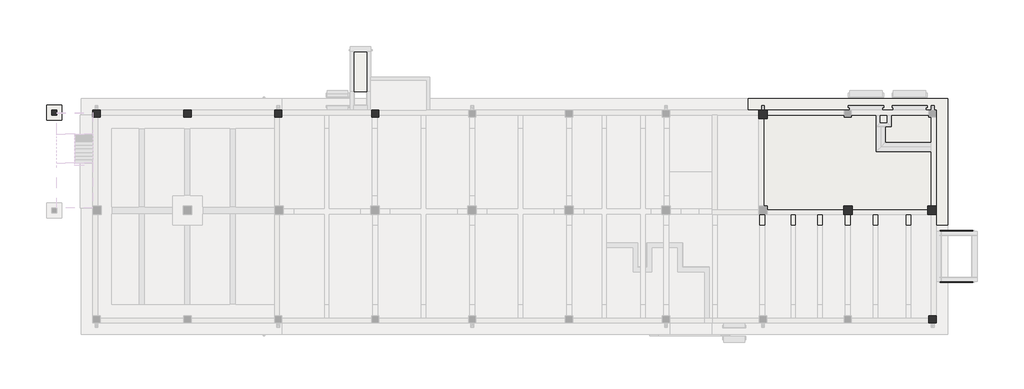
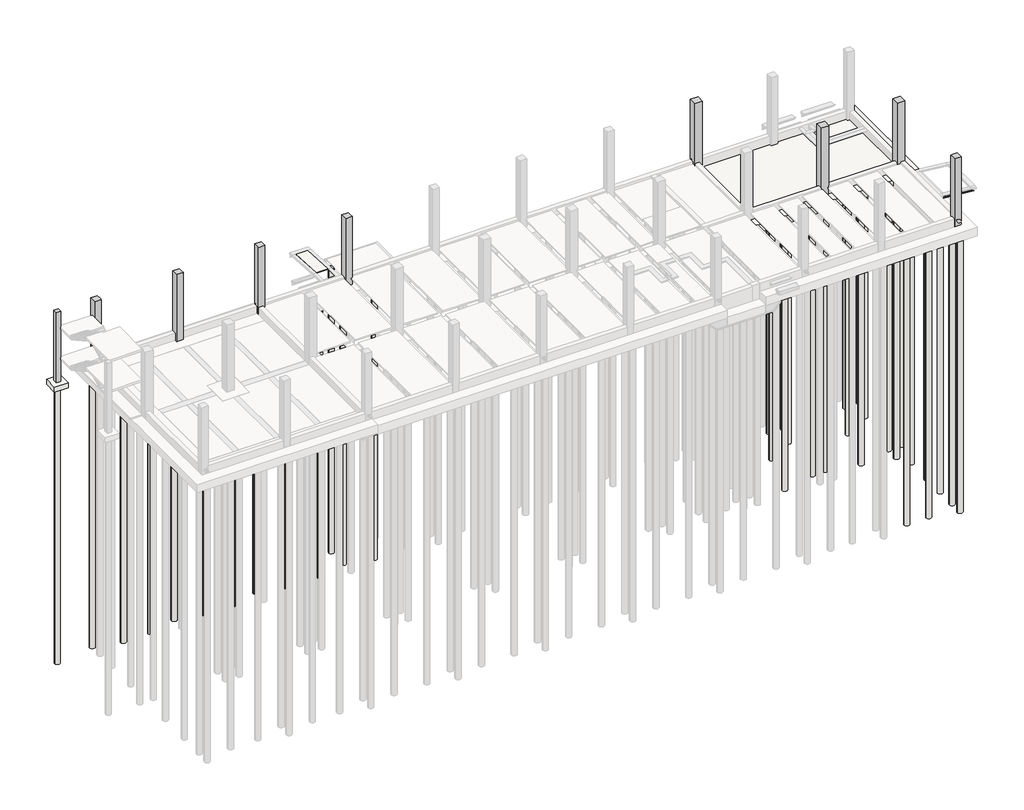
# One storey, part 6 of 7: 46 slabs, 9 columns.
"""IFC4 building model written with IfcOpenShell, lengths in millimetres."""

from ifc_helpers import new_model, si_unit, point, frame, frame_2d, origin, place, context, project, spatial, polyline, circle_curve, trimmed, segment, composite_curve, outline, extrude, faceted_brep, element, save

model = new_model("IFC4")

# Units and contexts
model_context = context("Model", 3, world=origin())
ifc_project = project(units=[si_unit("LENGTHUNIT", "METRE", prefix="MILLI")], contexts=[model_context])

# Site, building, storey
site = spatial("IfcSite", under=ifc_project)
building = spatial("IfcBuilding", under=site)
storey = spatial("IfcBuildingStorey", under=building, Name="H.P.P", Elevation=4500.0)

# Columns
placement = place(None, origin())
element("IfcColumn", 1, ObjectType="RC_Column_Rectangular : H_SC_AR S15_RC Col-AG_700x700_C1", at=placement, inside=storey, context=model_context, shape_type="Brep", body=[
    faceted_brep([(62350.0, -7650.0, 4000.0), (62350.0, -7950.0, 4000.0), (62350.0, -8350.0, 4000.0), (61650.0, -8350.0, 4000.0), (61650.0, -7950.0, 4000.0), (61650.0, -7650.0, 4000.0), (62350.0, -7650.0, 10600.0), (62350.0, -8350.0, 10600.0), (62350.0, -8350.0, 10450.0), (62350.0, -8350.0, 9800.0), (62350.0, -8350.0, 4800.0), (62350.0, -8350.0, 4650.0), (62250.0, -8350.0, 10600.0), (61750.0, -8350.0, 10600.0), (61650.0, -8350.0, 10600.0), (61650.0, -8350.0, 10450.0), (61650.0, -8350.0, 9800.0), (61650.0, -8350.0, 4800.0), (61650.0, -8350.0, 4650.0), (61650.0, -7650.0, 10600.0)], [[[0, 1, 2, 3, 4, 5]], [[2, 1, 0, 6, 7, 8, 9, 10, 11]], [[3, 2, 11, 10, 9, 8, 7, 12, 13, 14, 15, 16, 17, 18]], [[5, 4, 3, 18, 17, 16, 15, 14, 19]], [[0, 5, 19, 6]], [[7, 6, 19, 14, 13, 12]]]),
])
element("IfcColumn", 2, ObjectType="RC_Column_Rectangular : H_SC_AR S15_RC Col-AG_700x700_C1", at=placement, inside=storey, context=model_context, shape_type="Brep", body=[
    faceted_brep([(69300.0, -7650.0, 4000.0), (69300.0, -8350.0, 4000.0), (68900.0, -8350.0, 4000.0), (68600.0, -8350.0, 4000.0), (68600.0, -7950.0, 4000.0), (68600.0, -7650.0, 4000.0), (68900.0, -7650.0, 4000.0), (69300.0, -7650.0, 4800.0), (69300.0, -7650.0, 9900.0), (69300.0, -7650.0, 10600.0), (69300.0, -8350.0, 10600.0), (69300.0, -8350.0, 9900.0), (69300.0, -8350.0, 4800.0), (68900.0, -8350.0, 10600.0), (68600.0, -8350.0, 10600.0), (68600.0, -8350.0, 10450.0), (68600.0, -8350.0, 9800.0), (68600.0, -8350.0, 4800.0), (68600.0, -8350.0, 4650.0), (68600.0, -7650.0, 10600.0), (68900.0, -7650.0, 10600.0)], [[[0, 1, 2, 3, 4, 5, 6]], [[1, 0, 7, 8, 9, 10, 11, 12]], [[3, 2, 1, 12, 11, 10, 13, 14, 15, 16, 17, 18]], [[5, 4, 3, 18, 17, 16, 15, 14, 19]], [[0, 6, 5, 19, 20, 9, 8, 7]], [[10, 9, 20, 19, 14, 13]]]),
])
element("IfcColumn", 3, ObjectType="RC_Column_Rectangular : H_SC_AR S15_RC Col-AG_700x700_C1", at=placement, inside=storey, context=model_context, shape_type="Brep", body=[
    faceted_brep([(55350.0, 300.0, 4000.0), (55350.0, -100.0, 4000.0), (55350.0, -400.0, 4000.0), (55050.0, -400.0, 4000.0), (54650.0, -400.0, 4000.0), (54650.0, -100.0, 4000.0), (54650.0, 300.0, 4000.0), (55350.0, 300.0, 10600.0), (55350.0, -400.0, 10600.0), (55350.0, 300.0, 4800.0), (55350.0, 300.0, 8300.0), (55350.0, 300.0, 9100.0), (54650.0, -400.0, 10600.0), (54650.0, -400.0, 9800.0), (54650.0, -400.0, 4800.0), (54650.0, 300.0, 10600.0), (54650.0, 300.0, 9800.0), (54650.0, 300.0, 4800.0)], [[[0, 1, 2, 3, 4, 5, 6]], [[7, 8, 2, 1, 0, 9, 10, 11]], [[8, 12, 13, 14, 4, 3, 2]], [[12, 15, 16, 17, 6, 5, 4, 14, 13]], [[15, 7, 11, 10, 9, 0, 6, 17, 16]], [[7, 15, 12, 8]]]),
])
element("IfcColumn", 4, ObjectType="RC_Column_Rectangular : H_SC_AR S15_RC Col-AG_600x600_C2", at=placement, inside=storey, context=model_context, shape_type="Brep", body=[
    faceted_brep([(300.0, 300.0, 4100.0), (300.0, -100.0, 4100.0), (300.0, -300.0, 4100.0), (100.0, -300.0, 4100.0), (-300.0, -300.0, 4100.0), (-300.0, -100.0, 4100.0), (-300.0, 300.0, 4100.0), (300.0, 300.0, 4800.0), (300.0, 300.0, 9800.0), (300.0, 300.0, 10600.0), (300.0, -100.0, 10600.0), (300.0, -300.0, 10600.0), (300.0, -300.0, 10450.0), (100.0, -300.0, 10600.0), (-300.0, -300.0, 10600.0), (-300.0, -300.0, 9900.0), (-300.0, -300.0, 4800.0), (-300.0, 300.0, 10600.0), (-300.0, 300.0, 10550.0), (-300.0, 300.0, 9950.0), (-300.0, 300.0, 4630.0)], [[[0, 1, 2, 3, 4, 5, 6]], [[2, 1, 0, 7, 8, 9, 10, 11, 12]], [[4, 3, 2, 12, 11, 13, 14, 15, 16]], [[6, 5, 4, 16, 15, 14, 17, 18, 19, 20]], [[0, 6, 20, 19, 18, 17, 9, 8, 7]], [[17, 14, 13, 11, 10, 9]]]),
])
element("IfcColumn", 5, ObjectType="RC_Column_Rectangular : H_SC_AR S15_RC Col-AG_600x600_C2", at=placement, inside=storey, context=model_context, shape_type="Brep", body=[
    faceted_brep([(7800.0, 300.0, 4100.0), (7800.0, -100.0, 4100.0), (7800.0, -300.0, 4100.0), (7200.0, -300.0, 4100.0), (7200.0, -100.0, 4100.0), (7200.0, 300.0, 4100.0), (7800.0, 300.0, 4800.0), (7800.0, 300.0, 9800.0), (7800.0, 300.0, 10600.0), (7800.0, -100.0, 10600.0), (7800.0, -300.0, 10600.0), (7800.0, -300.0, 10450.0), (7750.0, -300.0, 10600.0), (7250.0, -300.0, 10600.0), (7200.0, -300.0, 10600.0), (7200.0, -300.0, 10450.0), (7200.0, -100.0, 10600.0), (7200.0, 300.0, 10600.0), (7200.0, 300.0, 9800.0), (7200.0, 300.0, 4800.0)], [[[0, 1, 2, 3, 4, 5]], [[2, 1, 0, 6, 7, 8, 9, 10, 11]], [[3, 2, 11, 10, 12, 13, 14, 15]], [[5, 4, 3, 15, 14, 16, 17, 18, 19]], [[0, 5, 19, 18, 17, 8, 7, 6]], [[8, 17, 16, 14, 13, 12, 10, 9]]]),
])
element("IfcColumn", 6, ObjectType="RC_Column_Rectangular : H_SC_AR S15_RC Col-AG_600x600_C2", at=placement, inside=storey, context=model_context, shape_type="Brep", body=[
    faceted_brep([(15300.0, 300.0, 4100.0), (15300.0, -300.0, 4100.0), (15100.0, -300.0, 4100.0), (14700.0, -300.0, 4100.0), (14700.0, -100.0, 4100.0), (14700.0, 300.0, 4100.0), (15300.0, 300.0, 4800.0), (15300.0, 300.0, 9800.0), (15300.0, 300.0, 10600.0), (15300.0, -100.0, 10600.0), (15300.0, -300.0, 10600.0), (15300.0, -300.0, 10450.0), (15300.0, -300.0, 4800.0), (15300.0, -300.0, 4650.0), (15200.0, -300.0, 10600.0), (14700.0, -300.0, 10600.0), (14700.0, -300.0, 10450.0), (14700.0, -300.0, 4800.0), (14700.0, -100.0, 10600.0), (14700.0, 300.0, 10600.0), (14700.0, 300.0, 9800.0), (14700.0, 300.0, 4800.0)], [[[0, 1, 2, 3, 4, 5]], [[1, 0, 6, 7, 8, 9, 10, 11, 12, 13]], [[3, 2, 1, 13, 12, 11, 10, 14, 15, 16, 17]], [[5, 4, 3, 17, 16, 15, 18, 19, 20, 21]], [[0, 5, 21, 20, 19, 8, 7, 6]], [[8, 19, 18, 15, 14, 10, 9]]]),
])
element("IfcColumn", 7, ObjectType="RC_Column_Rectangular : H_SC_AR S15_RC Col-AG_600x600_C2", at=placement, inside=storey, context=model_context, shape_type="Brep", body=[
    faceted_brep([(23300.0, 300.0, 4000.0), (23300.0, -100.0, 4000.0), (23300.0, -300.0, 4000.0), (22700.0, -300.0, 4000.0), (22700.0, -100.0, 4000.0), (22700.0, 300.0, 4000.0), (23300.0, 300.0, 4800.0), (23300.0, 300.0, 9800.0), (23300.0, 300.0, 10600.0), (23300.0, -100.0, 10600.0), (23300.0, -300.0, 10600.0), (23300.0, -300.0, 10450.0), (23300.0, -300.0, 4800.0), (23300.0, -300.0, 4650.0), (23200.0, -300.0, 10600.0), (22700.0, -300.0, 10600.0), (22700.0, -300.0, 10450.0), (22700.0, -300.0, 4800.0), (22700.0, -300.0, 4650.0), (22700.0, -100.0, 10600.0), (22700.0, 300.0, 10600.0), (22700.0, 300.0, 4800.0)], [[[0, 1, 2, 3, 4, 5]], [[2, 1, 0, 6, 7, 8, 9, 10, 11, 12, 13]], [[3, 2, 13, 12, 11, 10, 14, 15, 16, 17, 18]], [[5, 4, 3, 18, 17, 16, 15, 19, 20, 21]], [[0, 5, 21, 20, 8, 7, 6]], [[8, 20, 19, 15, 14, 10, 9]]]),
])
element("IfcColumn", 8, ObjectType="RC_Column_Rectangular : H_SC_AR S15_RC Col-AG_600x600_C2", at=placement, inside=storey, context=model_context, shape_type="Brep", body=[
    faceted_brep([(69300.0, -16700.0, 4000.0), (69300.0, -17300.0, 4000.0), (68700.0, -17300.0, 4000.0), (68700.0, -16900.0, 4000.0), (68700.0, -16700.0, 4000.0), (68900.0, -16700.0, 4000.0), (69300.0, -16700.0, 4800.0), (69300.0, -16700.0, 9900.0), (69300.0, -16700.0, 10600.0), (69300.0, -17300.0, 10600.0), (68700.0, -17300.0, 10600.0), (68700.0, -17300.0, 9800.0), (68700.0, -17300.0, 4800.0), (68700.0, -16900.0, 10600.0), (68700.0, -16700.0, 10600.0), (68700.0, -16700.0, 10450.0), (68700.0, -16700.0, 4800.0), (68700.0, -16700.0, 4650.0), (68900.0, -16700.0, 10600.0)], [[[0, 1, 2, 3, 4, 5]], [[1, 0, 6, 7, 8, 9]], [[2, 1, 9, 10, 11, 12]], [[4, 3, 2, 12, 11, 10, 13, 14, 15, 16, 17]], [[0, 5, 4, 17, 16, 15, 14, 18, 8, 7, 6]], [[9, 8, 18, 14, 13, 10]]]),
])
element("IfcColumn", 9, ObjectType="RC_Column_Rectangular : H_SC_AR S15_RC Col-AG_400x400_C3", at=placement, inside=storey, context=model_context, shape_type="Brep", body=[
    faceted_brep([(-3300.0, 300.0, 3800.0), (-3300.0, -100.0, 3800.0), (-3700.0, -100.0, 3800.0), (-3700.0, 300.0, 3800.0), (-3300.0, 300.0, 10600.0), (-3300.0, -100.0, 10600.0), (-3300.0, -100.0, 10550.0), (-3300.0, -100.0, 9950.0), (-3300.0, -100.0, 7590.0), (-3300.0, -100.0, 6990.0), (-3300.0, -100.0, 4630.0), (-3300.0, -100.0, 4100.0), (-3300.0, -100.0, 4030.0), (-3300.0, 300.0, 4100.0), (-3300.0, 300.0, 4630.0), (-3300.0, 300.0, 9950.0), (-3300.0, 300.0, 10550.0), (-3700.0, -100.0, 10600.0), (-3700.0, -100.0, 10550.0), (-3700.0, -100.0, 9950.0), (-3700.0, -100.0, 7590.0), (-3700.0, -100.0, 6990.0), (-3700.0, -100.0, 4630.0), (-3700.0, -100.0, 4030.0), (-3700.0, 300.0, 10600.0)], [[[0, 1, 2, 3]], [[4, 5, 6, 7, 8, 9, 10, 11, 12, 1, 0, 13, 14, 15, 16]], [[5, 17, 18, 19, 20, 21, 22, 23, 2, 1, 12, 11, 10, 9, 8, 7, 6]], [[17, 24, 3, 2, 23, 22, 21, 20, 19, 18]], [[24, 4, 16, 15, 14, 13, 0, 3]], [[4, 24, 17, 5]]]),
])

# Slabs
element("IfcSlab", 10, ObjectType="H_SF_AR S18_MAT_T800_MF1", at=placement, inside=storey, context=model_context, shape_type="Brep", body=[
    faceted_brep([(70250.0, 1249.9999999, 3200.0), (70250.0, -9250.0000001, 3200.0), (67750.0000002, -9250.0000001, 3200.0), (53749.9998007, -9250.0000001, 3200.0), (53749.9998007, -6750.0000001, 3200.0), (53749.9998007, -1250.0000001, 3200.0), (53749.9998007, 1249.9999999, 3200.0), (70250.0, -9250.0000001, 4000.0), (70250.0, 1249.9999999, 4000.0), (53749.9998007, 1249.9999999, 4000.0), (53749.9998007, -1250.0000001, 4000.0), (53749.9998007, -6750.0000001, 4000.0), (53749.9998007, -9250.0000001, 4000.0), (67750.0000002, -9250.0000001, 4000.0)], [[[0, 1, 2, 3, 4, 5, 6]], [[7, 8, 9, 10, 11, 12, 13]], [[1, 0, 8, 7]], [[1, 7, 13, 12, 3, 2]], [[3, 12, 11, 10, 9, 6, 5, 4]], [[0, 6, 9, 8]]]),
])
element("IfcSlab", 11, ObjectType="H_SF_AR_S18_Lean_T50", at=placement, inside=storey, context=model_context, shape_type="Brep", body=[
    faceted_brep([(72401.1499651, -13950.0, 4178.1393567), (69580.8773013, -13950.0, 4460.1666231), (69580.8773013, -13700.0, 4460.1666231), (72401.1499651, -13700.0, 4178.1393567), (69626.5585541, -13700.0, 4505.847876), (69626.5585541, -13850.0, 4505.847876), (69626.5585541, -13950.0, 4505.847876), (72345.3173228, -13950.0, 4233.9719991), (72345.3173228, -13850.0, 4233.9719991), (72345.3173228, -13700.0, 4233.9719991)], [[[0, 1, 2, 3]], [[4, 5, 6, 7, 8, 9]], [[1, 0, 7, 6]], [[3, 2, 4, 9]], [[5, 4, 2, 1, 6]], [[0, 3, 9, 8, 7]]]),
])
element("IfcSlab", 12, ObjectType="H_SF_AR_S18_Lean_T50", at=placement, inside=storey, context=model_context, shape_type="Brep", body=[
    faceted_brep([(69580.8773013, -9650.0, 4460.1666231), (72401.1499651, -9650.0, 4178.1393567), (72401.1499651, -9900.0, 4178.1393567), (69580.8773013, -9900.0, 4460.1666231), (72345.3173228, -9750.0, 4233.9719991), (72345.3173228, -9650.0, 4233.9719991), (69626.5585541, -9650.0, 4505.847876), (69626.5585541, -9750.0, 4505.847876), (69626.5585541, -9900.0, 4505.847876), (72345.3173228, -9900.0, 4233.9719991)], [[[0, 1, 2, 3]], [[4, 5, 6, 7, 8, 9]], [[1, 0, 6, 5]], [[3, 2, 9, 8]], [[2, 1, 5, 4, 9]], [[0, 3, 8, 7, 6]]]),
])
element("IfcSlab", 13, ObjectType="H_SF_AR_S18_Lean_T50", at=placement, inside=storey, context=model_context, shape_type="Brep", body=[
    faceted_brep([(22338.0, 5100.0, 4329.5560483), (22338.0, 1800.0, 4549.5560483), (21238.0, 1800.0, 4549.5560483), (21238.0, 5100.0, 4329.5560483), (22338.0, 5100.0, 4379.6670362), (21238.0, 5100.0, 4379.6670362), (21238.0, 1800.0, 4599.6670362), (22338.0, 1800.0, 4599.6670362), (22338.0, 1800.0, 4550.0), (21238.0, 1800.0, 4550.0)], [[[0, 1, 2, 3]], [[4, 5, 6, 7]], [[1, 0, 4, 7, 8]], [[2, 1, 8, 7, 6, 9]], [[3, 2, 9, 6, 5]], [[0, 3, 5, 4]]]),
])
element("IfcSlab", 14, ObjectType="Foundation Rectangular (Non-Pile) : H_SF_AR S18_Ret Fdn_1250x1250xT500_F2", at=placement, inside=storey, context=model_context, shape_type="SweptSolid", body=[
    extrude(outline(polyline([(-2875.0, 725.0), (-2875.0, -525.0), (-4125.0, -525.0), (-4125.0, 725.0), (-2875.0, 725.0)])), frame((0.0, 0.0, 3300.0), z_axis=(0.0, 0.0, 1.0), x_axis=(1.0, 0.0, 0.0)), (0.0, 0.0, 1.0), 500.0),
])
element("IfcSlab", 15, ObjectType="PILE : H_FL_AR S19_Pile_D500_L26.9", at=placement, inside=storey, context=model_context, shape_type="SweptSolid", body=[
    extrude(outline(composite_curve([segment(trimmed(circle_curve(frame_2d((-3500.0, 100.0)), 250.0), [point((-3250.0, 100.0))], [point((-3750.0, 100.0))], False, "CARTESIAN"), True, "CONTINUOUS"), segment(trimmed(circle_curve(frame_2d((-3500.0, 100.0)), 250.0), [point((-3750.0, 100.0))], [point((-3250.0, 100.0))], False, "CARTESIAN"), True, "CONTINUOUS")], self_intersect=False)), frame((0.0, 0.0, 3300.0), z_axis=(0.0, 0.0, 1.0), x_axis=(1.0, 0.0, 0.0)), (0.0, 0.0, 1.0), 100.0),
    extrude(outline(composite_curve([segment(trimmed(circle_curve(frame_2d((-3500.0, 100.0)), 250.0), [point((-3750.0, 100.0))], [point((-3250.0, 100.0))], False, "CARTESIAN"), True, "CONTINUOUS"), segment(trimmed(circle_curve(frame_2d((-3500.0, 100.0)), 250.0), [point((-3250.0, 100.0))], [point((-3750.0, 100.0))], False, "CARTESIAN"), True, "CONTINUOUS")], self_intersect=False)), frame((0.0, 0.0, -23500.0), z_axis=(0.0, 0.0, 1.0), x_axis=(1.0, 0.0, 0.0)), (0.0, 0.0, 1.0), 26750.0),
])
element("IfcSlab", 16, ObjectType="PILE : H_FL_AR S19_Pile_D500_L26.9", at=placement, inside=storey, context=model_context, shape_type="SweptSolid", body=[
    extrude(outline(composite_curve([segment(trimmed(circle_curve(frame_2d((0.0, 624.9999997)), 250.0), [point((-250.0, 624.9999997))], [point((250.0, 624.9999997))], False, "CARTESIAN"), True, "CONTINUOUS"), segment(trimmed(circle_curve(frame_2d((0.0, 624.9999997)), 250.0), [point((250.0, 624.9999997))], [point((-250.0, 624.9999997))], False, "CARTESIAN"), True, "CONTINUOUS")], self_intersect=False)), frame((0.0, 0.0, -23500.0), z_axis=(0.0, 0.0, 1.0), x_axis=(1.0, 0.0, 0.0)), (0.0, 0.0, 1.0), 26750.0),
])
element("IfcSlab", 17, ObjectType="PILE : H_FL_AR S19_Pile_D500_L26.9", at=placement, inside=storey, context=model_context, shape_type="SweptSolid", body=[
    extrude(outline(composite_curve([segment(trimmed(circle_curve(frame_2d((2500.0000001, 0.0)), 250.0), [point((2250.0000001, 0.0))], [point((2750.0000001, 0.0))], False, "CARTESIAN"), True, "CONTINUOUS"), segment(trimmed(circle_curve(frame_2d((2500.0000001, 0.0)), 250.0), [point((2750.0000001, 0.0))], [point((2250.0000001, 0.0))], False, "CARTESIAN"), True, "CONTINUOUS")], self_intersect=False)), frame((0.0, 0.0, -23500.0), z_axis=(0.0, 0.0, 1.0), x_axis=(1.0, 0.0, 0.0)), (0.0, 0.0, 1.0), 26750.0),
])
element("IfcSlab", 18, ObjectType="PILE : H_FL_AR S19_Pile_D500_L26.9", at=placement, inside=storey, context=model_context, shape_type="SweptSolid", body=[
    extrude(outline(composite_curve([segment(trimmed(circle_curve(frame_2d((5000.0000002, 0.0)), 250.0), [point((4750.0000002, 0.0))], [point((5250.0000002, 0.0))], False, "CARTESIAN"), True, "CONTINUOUS"), segment(trimmed(circle_curve(frame_2d((5000.0000002, 0.0)), 250.0), [point((5250.0000002, 0.0))], [point((4750.0000002, 0.0))], False, "CARTESIAN"), True, "CONTINUOUS")], self_intersect=False)), frame((0.0, 0.0, -23500.0), z_axis=(0.0, 0.0, 1.0), x_axis=(1.0, 0.0, 0.0)), (0.0, 0.0, 1.0), 26750.0),
])
element("IfcSlab", 19, ObjectType="PILE : H_FL_AR S19_Pile_D500_L26.9", at=placement, inside=storey, context=model_context, shape_type="SweptSolid", body=[
    extrude(outline(composite_curve([segment(trimmed(circle_curve(frame_2d((7500.0, 625.0)), 250.0), [point((7250.0, 625.0))], [point((7750.0, 625.0))], False, "CARTESIAN"), True, "CONTINUOUS"), segment(trimmed(circle_curve(frame_2d((7500.0, 625.0)), 250.0), [point((7750.0, 625.0))], [point((7250.0, 625.0))], False, "CARTESIAN"), True, "CONTINUOUS")], self_intersect=False)), frame((0.0, 0.0, -23500.0), z_axis=(0.0, 0.0, 1.0), x_axis=(1.0, 0.0, 0.0)), (0.0, 0.0, 1.0), 26750.0),
])
element("IfcSlab", 20, ObjectType="PILE : H_FL_AR S19_Pile_D500_L26.9", at=placement, inside=storey, context=model_context, shape_type="SweptSolid", body=[
    extrude(outline(composite_curve([segment(trimmed(circle_curve(frame_2d((10000.0000005, 0.0)), 250.0), [point((9750.0000005, 0.0))], [point((10250.0000005, 0.0))], False, "CARTESIAN"), True, "CONTINUOUS"), segment(trimmed(circle_curve(frame_2d((10000.0000005, 0.0)), 250.0), [point((10250.0000005, 0.0))], [point((9750.0000005, 0.0))], False, "CARTESIAN"), True, "CONTINUOUS")], self_intersect=False)), frame((0.0, 0.0, -23500.0), z_axis=(0.0, 0.0, 1.0), x_axis=(1.0, 0.0, 0.0)), (0.0, 0.0, 1.0), 26750.0),
])
element("IfcSlab", 21, ObjectType="PILE : H_FL_AR S19_Pile_D500_L26.9", at=placement, inside=storey, context=model_context, shape_type="SweptSolid", body=[
    extrude(outline(composite_curve([segment(trimmed(circle_curve(frame_2d((12500.0000007, 0.0)), 250.0), [point((12250.0000007, 0.0))], [point((12750.0000007, 0.0))], False, "CARTESIAN"), True, "CONTINUOUS"), segment(trimmed(circle_curve(frame_2d((12500.0000007, 0.0)), 250.0), [point((12750.0000007, 0.0))], [point((12250.0000007, 0.0))], False, "CARTESIAN"), True, "CONTINUOUS")], self_intersect=False)), frame((0.0, 0.0, -23500.0), z_axis=(0.0, 0.0, 1.0), x_axis=(1.0, 0.0, 0.0)), (0.0, 0.0, 1.0), 26750.0),
])
element("IfcSlab", 22, ObjectType="PILE : H_FL_AR S19_Pile_D500_L26.8", at=placement, inside=storey, context=model_context, shape_type="SweptSolid", body=[
    extrude(outline(composite_curve([segment(trimmed(circle_curve(frame_2d((14999.9999999, 625.0000001)), 250.0), [point((15249.9999999, 625.0000001))], [point((14749.9999999, 625.0000001))], False, "CARTESIAN"), True, "CONTINUOUS"), segment(trimmed(circle_curve(frame_2d((14999.9999999, 625.0000001)), 250.0), [point((14749.9999999, 625.0000001))], [point((15249.9999999, 625.0000001))], False, "CARTESIAN"), True, "CONTINUOUS")], self_intersect=False)), frame((0.0, 0.0, 3200.0), z_axis=(0.0, 0.0, 1.0), x_axis=(1.0, 0.0, 0.0)), (0.0, 0.0, 1.0), 100.0),
    extrude(outline(composite_curve([segment(trimmed(circle_curve(frame_2d((14999.9999999, 625.0000001)), 250.0), [point((14749.9999999, 625.0000001))], [point((15249.9999999, 625.0000001))], False, "CARTESIAN"), True, "CONTINUOUS"), segment(trimmed(circle_curve(frame_2d((14999.9999999, 625.0000001)), 250.0), [point((15249.9999999, 625.0000001))], [point((14749.9999999, 625.0000001))], False, "CARTESIAN"), True, "CONTINUOUS")], self_intersect=False)), frame((0.0, 0.0, -23500.0), z_axis=(0.0, 0.0, 1.0), x_axis=(1.0, 0.0, 0.0)), (0.0, 0.0, 1.0), 26650.0),
])
element("IfcSlab", 23, ObjectType="PILE : H_FL_AR S19_Pile_D500_L26.8", at=placement, inside=storey, context=model_context, shape_type="SweptSolid", body=[
    extrude(outline(composite_curve([segment(trimmed(circle_curve(frame_2d((17500.0000007, 0.0)), 250.0), [point((17250.0000007, 0.0))], [point((17750.0000007, 0.0))], False, "CARTESIAN"), True, "CONTINUOUS"), segment(trimmed(circle_curve(frame_2d((17500.0000007, 0.0)), 250.0), [point((17750.0000007, 0.0))], [point((17250.0000007, 0.0))], False, "CARTESIAN"), True, "CONTINUOUS")], self_intersect=False)), frame((0.0, 0.0, -23500.0), z_axis=(0.0, 0.0, 1.0), x_axis=(1.0, 0.0, 0.0)), (0.0, 0.0, 1.0), 26650.0),
])
element("IfcSlab", 24, ObjectType="PILE : H_FL_AR S19_Pile_D500_L26.8", at=placement, inside=storey, context=model_context, shape_type="SweptSolid", body=[
    extrude(outline(composite_curve([segment(trimmed(circle_curve(frame_2d((20499.9999999, 0.0)), 250.0), [point((20249.9999999, 0.0))], [point((20749.9999999, 0.0))], False, "CARTESIAN"), True, "CONTINUOUS"), segment(trimmed(circle_curve(frame_2d((20499.9999999, 0.0)), 250.0), [point((20749.9999999, 0.0))], [point((20249.9999999, 0.0))], False, "CARTESIAN"), True, "CONTINUOUS")], self_intersect=False)), frame((0.0, 0.0, -23500.0), z_axis=(0.0, 0.0, 1.0), x_axis=(1.0, 0.0, 0.0)), (0.0, 0.0, 1.0), 26650.0),
])
element("IfcSlab", 25, ObjectType="PILE : H_FL_AR S19_Pile_D500_L26.8", at=placement, inside=storey, context=model_context, shape_type="SweptSolid", body=[
    extrude(outline(composite_curve([segment(trimmed(circle_curve(frame_2d((23000.0, 624.9999997)), 250.0), [point((22750.0, 624.9999997))], [point((23250.0, 624.9999997))], False, "CARTESIAN"), True, "CONTINUOUS"), segment(trimmed(circle_curve(frame_2d((23000.0, 624.9999997)), 250.0), [point((23250.0, 624.9999997))], [point((22750.0, 624.9999997))], False, "CARTESIAN"), True, "CONTINUOUS")], self_intersect=False)), frame((0.0, 0.0, -23500.0), z_axis=(0.0, 0.0, 1.0), x_axis=(1.0, 0.0, 0.0)), (0.0, 0.0, 1.0), 26650.0),
])
element("IfcSlab", 26, ObjectType="PILE : H_FL_AR S19_Pile_D500_L27.7", at=placement, inside=storey, context=model_context, shape_type="SweptSolid", body=[
    extrude(outline(composite_curve([segment(trimmed(circle_curve(frame_2d((23000.0, 2500.0)), 250.0), [point((22750.0, 2500.0))], [point((23250.0, 2500.0))], False, "CARTESIAN"), True, "CONTINUOUS"), segment(trimmed(circle_curve(frame_2d((23000.0, 2500.0)), 250.0), [point((23250.0, 2500.0))], [point((22750.0, 2500.0))], False, "CARTESIAN"), True, "CONTINUOUS")], self_intersect=False)), frame((0.0, 0.0, -23500.0), z_axis=(0.0, 0.0, 1.0), x_axis=(1.0, 0.0, 0.0)), (0.0, 0.0, 1.0), 27550.0),
])
element("IfcSlab", 27, ObjectType="PILE : H_FL_AR S19_Pile_D500_L26.8", at=placement, inside=storey, context=model_context, shape_type="SweptSolid", body=[
    extrude(outline(composite_curve([segment(trimmed(circle_curve(frame_2d((25500.0000013, 0.0)), 250.0), [point((25250.0000013, 0.0))], [point((25750.0000013, 0.0))], False, "CARTESIAN"), True, "CONTINUOUS"), segment(trimmed(circle_curve(frame_2d((25500.0000013, 0.0)), 250.0), [point((25750.0000013, 0.0))], [point((25250.0000013, 0.0))], False, "CARTESIAN"), True, "CONTINUOUS")], self_intersect=False)), frame((0.0, 0.0, -23500.0), z_axis=(0.0, 0.0, 1.0), x_axis=(1.0, 0.0, 0.0)), (0.0, 0.0, 1.0), 26650.0),
])
element("IfcSlab", 28, ObjectType="PILE : H_FL_AR S19_Pile_D500_L26.8", at=placement, inside=storey, context=model_context, shape_type="SweptSolid", body=[
    extrude(outline(composite_curve([segment(trimmed(circle_curve(frame_2d((64499.9999998, -17000.0)), 250.0), [point((64249.9999998, -17000.0))], [point((64749.9999998, -17000.0))], False, "CARTESIAN"), True, "CONTINUOUS"), segment(trimmed(circle_curve(frame_2d((64499.9999998, -17000.0)), 250.0), [point((64749.9999998, -17000.0))], [point((64249.9999998, -17000.0))], False, "CARTESIAN"), True, "CONTINUOUS")], self_intersect=False)), frame((0.0, 0.0, -23500.0), z_axis=(0.0, 0.0, 1.0), x_axis=(1.0, 0.0, 0.0)), (0.0, 0.0, 1.0), 26650.0),
])
element("IfcSlab", 29, ObjectType="PILE : H_FL_AR S19_Pile_D500_L26.8", at=placement, inside=storey, context=model_context, shape_type="SweptSolid", body=[
    extrude(outline(composite_curve([segment(trimmed(circle_curve(frame_2d((66500.0, -17000.0)), 250.0), [point((66250.0, -17000.0))], [point((66750.0, -17000.0))], False, "CARTESIAN"), True, "CONTINUOUS"), segment(trimmed(circle_curve(frame_2d((66500.0, -17000.0)), 250.0), [point((66750.0, -17000.0))], [point((66250.0, -17000.0))], False, "CARTESIAN"), True, "CONTINUOUS")], self_intersect=False)), frame((0.0, 0.0, -23500.0), z_axis=(0.0, 0.0, 1.0), x_axis=(1.0, 0.0, 0.0)), (0.0, 0.0, 1.0), 26650.0),
])
element("IfcSlab", 30, ObjectType="PILE : H_FL_AR S19_Pile_D500_L26.8", at=placement, inside=storey, context=model_context, shape_type="SweptSolid", body=[
    extrude(outline(composite_curve([segment(trimmed(circle_curve(frame_2d((69000.0, -17625.0000002)), 250.0), [point((68750.0, -17625.0000002))], [point((69250.0, -17625.0000002))], False, "CARTESIAN"), True, "CONTINUOUS"), segment(trimmed(circle_curve(frame_2d((69000.0, -17625.0000002)), 250.0), [point((69250.0, -17625.0000002))], [point((68750.0, -17625.0000002))], False, "CARTESIAN"), True, "CONTINUOUS")], self_intersect=False)), frame((0.0, 0.0, -23500.0), z_axis=(0.0, 0.0, 1.0), x_axis=(1.0, 0.0, 0.0)), (0.0, 0.0, 1.0), 26650.0),
])
element("IfcSlab", 31, ObjectType="PILE : H_FL_AR S19_Pile_D500_L26.8", at=placement, inside=storey, context=model_context, shape_type="SweptSolid", body=[
    extrude(outline(composite_curve([segment(trimmed(circle_curve(frame_2d((69000.0, -16375.0000006)), 250.0), [point((68750.0, -16375.0000006))], [point((69250.0, -16375.0000006))], False, "CARTESIAN"), True, "CONTINUOUS"), segment(trimmed(circle_curve(frame_2d((69000.0, -16375.0000006)), 250.0), [point((69250.0, -16375.0000006))], [point((68750.0, -16375.0000006))], False, "CARTESIAN"), True, "CONTINUOUS")], self_intersect=False)), frame((0.0, 0.0, -23500.0), z_axis=(0.0, 0.0, 1.0), x_axis=(1.0, 0.0, 0.0)), (0.0, 0.0, 1.0), 26650.0),
])
element("IfcSlab", 32, ObjectType="PILE : H_FL_AR S19_Pile_D500_L26.8", at=placement, inside=storey, context=model_context, shape_type="SweptSolid", body=[
    extrude(outline(composite_curve([segment(trimmed(circle_curve(frame_2d((69000.0, -14499.9999999)), 250.0), [point((68750.0, -14499.9999999))], [point((69250.0, -14499.9999999))], False, "CARTESIAN"), True, "CONTINUOUS"), segment(trimmed(circle_curve(frame_2d((69000.0, -14499.9999999)), 250.0), [point((69250.0, -14499.9999999))], [point((68750.0, -14499.9999999))], False, "CARTESIAN"), True, "CONTINUOUS")], self_intersect=False)), frame((0.0, 0.0, -23500.0), z_axis=(0.0, 0.0, 1.0), x_axis=(1.0, 0.0, 0.0)), (0.0, 0.0, 1.0), 26650.0),
])
element("IfcSlab", 33, ObjectType="PILE : H_FL_AR S19_Pile_D500_L26.8", at=placement, inside=storey, context=model_context, shape_type="SweptSolid", body=[
    extrude(outline(composite_curve([segment(trimmed(circle_curve(frame_2d((69000.0, -12375.0000001)), 250.0), [point((68750.0, -12375.0000001))], [point((69250.0, -12375.0000001))], False, "CARTESIAN"), True, "CONTINUOUS"), segment(trimmed(circle_curve(frame_2d((69000.0, -12375.0000001)), 250.0), [point((69250.0, -12375.0000001))], [point((68750.0, -12375.0000001))], False, "CARTESIAN"), True, "CONTINUOUS")], self_intersect=False)), frame((0.0, 0.0, -23500.0), z_axis=(0.0, 0.0, 1.0), x_axis=(1.0, 0.0, 0.0)), (0.0, 0.0, 1.0), 26650.0),
])
element("IfcSlab", 34, ObjectType="PILE : H_FL_AR S19_Pile_D500_L26.8", at=placement, inside=storey, context=model_context, shape_type="SweptSolid", body=[
    extrude(outline(composite_curve([segment(trimmed(circle_curve(frame_2d((69000.0, -9874.9999999)), 250.0), [point((68750.0, -9874.9999999))], [point((69250.0, -9874.9999999))], False, "CARTESIAN"), True, "CONTINUOUS"), segment(trimmed(circle_curve(frame_2d((69000.0, -9874.9999999)), 250.0), [point((69250.0, -9874.9999999))], [point((68750.0, -9874.9999999))], False, "CARTESIAN"), True, "CONTINUOUS")], self_intersect=False)), frame((0.0, 0.0, -23500.0), z_axis=(0.0, 0.0, 1.0), x_axis=(1.0, 0.0, 0.0)), (0.0, 0.0, 1.0), 26650.0),
])
element("IfcSlab", 35, ObjectType="PILE : H_FL_AR S19_Pile_D500_L26.8", at=placement, inside=storey, context=model_context, shape_type="SweptSolid", body=[
    extrude(outline(composite_curve([segment(trimmed(circle_curve(frame_2d((69625.0, -8625.0)), 250.0), [point((69375.0, -8625.0))], [point((69875.0, -8625.0))], False, "CARTESIAN"), True, "CONTINUOUS"), segment(trimmed(circle_curve(frame_2d((69625.0, -8625.0)), 250.0), [point((69875.0, -8625.0))], [point((69375.0, -8625.0))], False, "CARTESIAN"), True, "CONTINUOUS")], self_intersect=False)), frame((0.0, 0.0, -23500.0), z_axis=(0.0, 0.0, 1.0), x_axis=(1.0, 0.0, 0.0)), (0.0, 0.0, 1.0), 26650.0),
])
element("IfcSlab", 36, ObjectType="PILE : H_FL_AR S19_Pile_D500_L26.8", at=placement, inside=storey, context=model_context, shape_type="SweptSolid", body=[
    extrude(outline(composite_curve([segment(trimmed(circle_curve(frame_2d((69625.0, -7375.0)), 250.0), [point((69375.0, -7375.0))], [point((69875.0, -7375.0))], False, "CARTESIAN"), True, "CONTINUOUS"), segment(trimmed(circle_curve(frame_2d((69625.0, -7375.0)), 250.0), [point((69875.0, -7375.0))], [point((69375.0, -7375.0))], False, "CARTESIAN"), True, "CONTINUOUS")], self_intersect=False)), frame((0.0, 0.0, -23500.0), z_axis=(0.0, 0.0, 1.0), x_axis=(1.0, 0.0, 0.0)), (0.0, 0.0, 1.0), 26650.0),
])
element("IfcSlab", 37, ObjectType="PILE : H_FL_AR S19_Pile_D500_L26.8", at=placement, inside=storey, context=model_context, shape_type="SweptSolid", body=[
    extrude(outline(composite_curve([segment(trimmed(circle_curve(frame_2d((68375.0, -7375.0)), 250.0), [point((68125.0, -7375.0))], [point((68625.0, -7375.0))], False, "CARTESIAN"), True, "CONTINUOUS"), segment(trimmed(circle_curve(frame_2d((68375.0, -7375.0)), 250.0), [point((68625.0, -7375.0))], [point((68125.0, -7375.0))], False, "CARTESIAN"), True, "CONTINUOUS")], self_intersect=False)), frame((0.0, 0.0, -23500.0), z_axis=(0.0, 0.0, 1.0), x_axis=(1.0, 0.0, 0.0)), (0.0, 0.0, 1.0), 26650.0),
])
element("IfcSlab", 38, ObjectType="PILE : H_FL_AR S19_Pile_D500_L26.8", at=placement, inside=storey, context=model_context, shape_type="SweptSolid", body=[
    extrude(outline(composite_curve([segment(trimmed(circle_curve(frame_2d((68375.0, -8625.0)), 250.0), [point((68125.0, -8625.0))], [point((68625.0, -8625.0))], False, "CARTESIAN"), True, "CONTINUOUS"), segment(trimmed(circle_curve(frame_2d((68375.0, -8625.0)), 250.0), [point((68625.0, -8625.0))], [point((68125.0, -8625.0))], False, "CARTESIAN"), True, "CONTINUOUS")], self_intersect=False)), frame((0.0, 0.0, -23500.0), z_axis=(0.0, 0.0, 1.0), x_axis=(1.0, 0.0, 0.0)), (0.0, 0.0, 1.0), 26650.0),
])
element("IfcSlab", 39, ObjectType="PILE : H_FL_AR S19_Pile_D500_L26.8", at=placement, inside=storey, context=model_context, shape_type="SweptSolid", body=[
    extrude(outline(composite_curve([segment(trimmed(circle_curve(frame_2d((65500.0, -8000.0)), 250.0), [point((65250.0, -8000.0))], [point((65750.0, -8000.0))], False, "CARTESIAN"), True, "CONTINUOUS"), segment(trimmed(circle_curve(frame_2d((65500.0, -8000.0)), 250.0), [point((65750.0, -8000.0))], [point((65250.0, -8000.0))], False, "CARTESIAN"), True, "CONTINUOUS")], self_intersect=False)), frame((0.0, 0.0, -23500.0), z_axis=(0.0, 0.0, 1.0), x_axis=(1.0, 0.0, 0.0)), (0.0, 0.0, 1.0), 26650.0),
])
element("IfcSlab", 40, ObjectType="PILE : H_FL_AR S19_Pile_D500_L26.8", at=placement, inside=storey, context=model_context, shape_type="SweptSolid", body=[
    extrude(outline(composite_curve([segment(trimmed(circle_curve(frame_2d((62625.0000001, -7375.0)), 250.0), [point((62375.0000001, -7375.0))], [point((62875.0000001, -7375.0))], False, "CARTESIAN"), True, "CONTINUOUS"), segment(trimmed(circle_curve(frame_2d((62625.0000001, -7375.0)), 250.0), [point((62875.0000001, -7375.0))], [point((62375.0000001, -7375.0))], False, "CARTESIAN"), True, "CONTINUOUS")], self_intersect=False)), frame((0.0, 0.0, -23500.0), z_axis=(0.0, 0.0, 1.0), x_axis=(1.0, 0.0, 0.0)), (0.0, 0.0, 1.0), 26650.0),
])
element("IfcSlab", 41, ObjectType="PILE : H_FL_AR S19_Pile_D500_L26.8", at=placement, inside=storey, context=model_context, shape_type="SweptSolid", body=[
    extrude(outline(composite_curve([segment(trimmed(circle_curve(frame_2d((61375.0000001, -7375.0)), 250.0), [point((61125.0000001, -7375.0))], [point((61625.0000001, -7375.0))], False, "CARTESIAN"), True, "CONTINUOUS"), segment(trimmed(circle_curve(frame_2d((61375.0000001, -7375.0)), 250.0), [point((61625.0000001, -7375.0))], [point((61125.0000001, -7375.0))], False, "CARTESIAN"), True, "CONTINUOUS")], self_intersect=False)), frame((0.0, 0.0, -23500.0), z_axis=(0.0, 0.0, 1.0), x_axis=(1.0, 0.0, 0.0)), (0.0, 0.0, 1.0), 26650.0),
])
element("IfcSlab", 42, ObjectType="PILE : H_FL_AR S19_Pile_D500_L26.8", at=placement, inside=storey, context=model_context, shape_type="SweptSolid", body=[
    extrude(outline(composite_curve([segment(trimmed(circle_curve(frame_2d((58500.0, -8000.0)), 250.0), [point((58250.0, -8000.0))], [point((58750.0, -8000.0))], False, "CARTESIAN"), True, "CONTINUOUS"), segment(trimmed(circle_curve(frame_2d((58500.0, -8000.0)), 250.0), [point((58750.0, -8000.0))], [point((58250.0, -8000.0))], False, "CARTESIAN"), True, "CONTINUOUS")], self_intersect=False)), frame((0.0, 0.0, -23500.0), z_axis=(0.0, 0.0, 1.0), x_axis=(1.0, 0.0, 0.0)), (0.0, 0.0, 1.0), 26650.0),
])
element("IfcSlab", 43, ObjectType="PILE : H_FL_AR S19_Pile_D500_L26.8", at=placement, inside=storey, context=model_context, shape_type="SweptSolid", body=[
    extrude(outline(composite_curve([segment(trimmed(circle_curve(frame_2d((57300.0, -3870.0)), 250.0), [point((57050.0, -3870.0))], [point((57550.0, -3870.0))], False, "CARTESIAN"), True, "CONTINUOUS"), segment(trimmed(circle_curve(frame_2d((57300.0, -3870.0)), 250.0), [point((57550.0, -3870.0))], [point((57050.0, -3870.0))], False, "CARTESIAN"), True, "CONTINUOUS")], self_intersect=False)), frame((0.0, 0.0, -23500.0), z_axis=(0.0, 0.0, 1.0), x_axis=(1.0, 0.0, 0.0)), (0.0, 0.0, 1.0), 26650.0),
])
element("IfcSlab", 44, ObjectType="PILE : H_FL_AR S19_Pile_D500_L26.8", at=placement, inside=storey, context=model_context, shape_type="SweptSolid", body=[
    extrude(outline(composite_curve([segment(trimmed(circle_curve(frame_2d((59700.0, -3870.0)), 250.0), [point((59450.0, -3870.0))], [point((59950.0, -3870.0))], False, "CARTESIAN"), True, "CONTINUOUS"), segment(trimmed(circle_curve(frame_2d((59700.0, -3870.0)), 250.0), [point((59950.0, -3870.0))], [point((59450.0, -3870.0))], False, "CARTESIAN"), True, "CONTINUOUS")], self_intersect=False)), frame((0.0, 0.0, -23500.0), z_axis=(0.0, 0.0, 1.0), x_axis=(1.0, 0.0, 0.0)), (0.0, 0.0, 1.0), 26650.0),
])
element("IfcSlab", 45, ObjectType="PILE : H_FL_AR S19_Pile_D500_L26.8", at=placement, inside=storey, context=model_context, shape_type="SweptSolid", body=[
    extrude(outline(composite_curve([segment(trimmed(circle_curve(frame_2d((62000.0, -5500.0)), 250.0), [point((61750.0, -5500.0))], [point((62250.0, -5500.0))], False, "CARTESIAN"), True, "CONTINUOUS"), segment(trimmed(circle_curve(frame_2d((62000.0, -5500.0)), 250.0), [point((62250.0, -5500.0))], [point((61750.0, -5500.0))], False, "CARTESIAN"), True, "CONTINUOUS")], self_intersect=False)), frame((0.0, 0.0, -23500.0), z_axis=(0.0, 0.0, 1.0), x_axis=(1.0, 0.0, 0.0)), (0.0, 0.0, 1.0), 26650.0),
])
element("IfcSlab", 46, ObjectType="PILE : H_FL_AR S19_Pile_D500_L26.8", at=placement, inside=storey, context=model_context, shape_type="SweptSolid", body=[
    extrude(outline(composite_curve([segment(trimmed(circle_curve(frame_2d((64300.0, -3870.0)), 250.0), [point((64050.0, -3870.0))], [point((64550.0, -3870.0))], False, "CARTESIAN"), True, "CONTINUOUS"), segment(trimmed(circle_curve(frame_2d((64300.0, -3870.0)), 250.0), [point((64550.0, -3870.0))], [point((64050.0, -3870.0))], False, "CARTESIAN"), True, "CONTINUOUS")], self_intersect=False)), frame((0.0, 0.0, -23500.0), z_axis=(0.0, 0.0, 1.0), x_axis=(1.0, 0.0, 0.0)), (0.0, 0.0, 1.0), 26650.0),
])
element("IfcSlab", 47, ObjectType="PILE : H_FL_AR S19_Pile_D500_L26.8", at=placement, inside=storey, context=model_context, shape_type="SweptSolid", body=[
    extrude(outline(composite_curve([segment(trimmed(circle_curve(frame_2d((62000.0, -2500.0000004)), 250.0), [point((61750.0, -2500.0000004))], [point((62250.0, -2500.0000004))], False, "CARTESIAN"), True, "CONTINUOUS"), segment(trimmed(circle_curve(frame_2d((62000.0, -2500.0000004)), 250.0), [point((62250.0, -2500.0000004))], [point((61750.0, -2500.0000004))], False, "CARTESIAN"), True, "CONTINUOUS")], self_intersect=False)), frame((0.0, 0.0, -23500.0), z_axis=(0.0, 0.0, 1.0), x_axis=(1.0, 0.0, 0.0)), (0.0, 0.0, 1.0), 26650.0),
])
element("IfcSlab", 48, ObjectType="PILE : H_FL_AR S19_Pile_D500_L26.8", at=placement, inside=storey, context=model_context, shape_type="SweptSolid", body=[
    extrude(outline(composite_curve([segment(trimmed(circle_curve(frame_2d((66700.0, -3870.0)), 250.0), [point((66450.0, -3870.0))], [point((66950.0, -3870.0))], False, "CARTESIAN"), True, "CONTINUOUS"), segment(trimmed(circle_curve(frame_2d((66700.0, -3870.0)), 250.0), [point((66950.0, -3870.0))], [point((66450.0, -3870.0))], False, "CARTESIAN"), True, "CONTINUOUS")], self_intersect=False)), frame((0.0, 0.0, -23500.0), z_axis=(0.0, 0.0, 1.0), x_axis=(1.0, 0.0, 0.0)), (0.0, 0.0, 1.0), 26650.0),
])
element("IfcSlab", 49, ObjectType="PILE : H_FL_AR S19_Pile_D500_L26.8", at=placement, inside=storey, context=model_context, shape_type="SweptSolid", body=[
    extrude(outline(composite_curve([segment(trimmed(circle_curve(frame_2d((69000.0, -5499.9999996)), 250.0), [point((68750.0, -5499.9999996))], [point((69250.0, -5499.9999996))], False, "CARTESIAN"), True, "CONTINUOUS"), segment(trimmed(circle_curve(frame_2d((69000.0, -5499.9999996)), 250.0), [point((69250.0, -5499.9999996))], [point((68750.0, -5499.9999996))], False, "CARTESIAN"), True, "CONTINUOUS")], self_intersect=False)), frame((0.0, 0.0, -23500.0), z_axis=(0.0, 0.0, 1.0), x_axis=(1.0, 0.0, 0.0)), (0.0, 0.0, 1.0), 26650.0),
])
element("IfcSlab", 50, ObjectType="PILE : H_FL_AR S19_Pile_D500_L26.8", at=placement, inside=storey, context=model_context, shape_type="SweptSolid", body=[
    extrude(outline(composite_curve([segment(trimmed(circle_curve(frame_2d((69000.0, -2500.0000004)), 250.0), [point((68750.0, -2500.0000004))], [point((69250.0, -2500.0000004))], False, "CARTESIAN"), True, "CONTINUOUS"), segment(trimmed(circle_curve(frame_2d((69000.0, -2500.0000004)), 250.0), [point((69250.0, -2500.0000004))], [point((68750.0, -2500.0000004))], False, "CARTESIAN"), True, "CONTINUOUS")], self_intersect=False)), frame((0.0, 0.0, -23500.0), z_axis=(0.0, 0.0, 1.0), x_axis=(1.0, 0.0, 0.0)), (0.0, 0.0, 1.0), 26650.0),
])
element("IfcSlab", 51, ObjectType="PILE : H_FL_AR S19_Pile_D500_L26.8", at=placement, inside=storey, context=model_context, shape_type="SweptSolid", body=[
    extrude(outline(composite_curve([segment(trimmed(circle_curve(frame_2d((69625.0, -625.0)), 250.0), [point((69375.0, -625.0))], [point((69875.0, -625.0))], False, "CARTESIAN"), True, "CONTINUOUS"), segment(trimmed(circle_curve(frame_2d((69625.0, -625.0)), 250.0), [point((69875.0, -625.0))], [point((69375.0, -625.0))], False, "CARTESIAN"), True, "CONTINUOUS")], self_intersect=False)), frame((0.0, 0.0, -23500.0), z_axis=(0.0, 0.0, 1.0), x_axis=(1.0, 0.0, 0.0)), (0.0, 0.0, 1.0), 26650.0),
])
element("IfcSlab", 52, ObjectType="PILE : H_FL_AR S19_Pile_D500_L26.8", at=placement, inside=storey, context=model_context, shape_type="SweptSolid", body=[
    extrude(outline(composite_curve([segment(trimmed(circle_curve(frame_2d((68375.0, -625.0)), 250.0), [point((68125.0, -625.0))], [point((68625.0, -625.0))], False, "CARTESIAN"), True, "CONTINUOUS"), segment(trimmed(circle_curve(frame_2d((68375.0, -625.0)), 250.0), [point((68625.0, -625.0))], [point((68125.0, -625.0))], False, "CARTESIAN"), True, "CONTINUOUS")], self_intersect=False)), frame((0.0, 0.0, -23500.0), z_axis=(0.0, 0.0, 1.0), x_axis=(1.0, 0.0, 0.0)), (0.0, 0.0, 1.0), 26650.0),
])
element("IfcSlab", 53, ObjectType="PILE : H_FL_AR S19_Pile_D500_L26.8", at=placement, inside=storey, context=model_context, shape_type="SweptSolid", body=[
    extrude(outline(composite_curve([segment(trimmed(circle_curve(frame_2d((62625.0000001, -625.0)), 250.0), [point((62375.0000001, -625.0))], [point((62875.0000001, -625.0))], False, "CARTESIAN"), True, "CONTINUOUS"), segment(trimmed(circle_curve(frame_2d((62625.0000001, -625.0)), 250.0), [point((62875.0000001, -625.0))], [point((62375.0000001, -625.0))], False, "CARTESIAN"), True, "CONTINUOUS")], self_intersect=False)), frame((0.0, 0.0, -23500.0), z_axis=(0.0, 0.0, 1.0), x_axis=(1.0, 0.0, 0.0)), (0.0, 0.0, 1.0), 26650.0),
])
element("IfcSlab", 54, ObjectType="PILE : H_FL_AR S19_Pile_D500_L26.8", at=placement, inside=storey, context=model_context, shape_type="SweptSolid", body=[
    extrude(outline(composite_curve([segment(trimmed(circle_curve(frame_2d((61375.0000001, -625.0)), 250.0), [point((61125.0000001, -625.0))], [point((61625.0000001, -625.0))], False, "CARTESIAN"), True, "CONTINUOUS"), segment(trimmed(circle_curve(frame_2d((61375.0000001, -625.0)), 250.0), [point((61625.0000001, -625.0))], [point((61125.0000001, -625.0))], False, "CARTESIAN"), True, "CONTINUOUS")], self_intersect=False)), frame((0.0, 0.0, -23500.0), z_axis=(0.0, 0.0, 1.0), x_axis=(1.0, 0.0, 0.0)), (0.0, 0.0, 1.0), 26650.0),
])
element("IfcSlab", 55, ObjectType="PILE : H_FL_AR S19_Pile_D500_L26.8", at=placement, inside=storey, context=model_context, shape_type="SweptSolid", body=[
    extrude(outline(composite_curve([segment(trimmed(circle_curve(frame_2d((55625.0, -625.0)), 250.0), [point((55375.0, -625.0))], [point((55875.0, -625.0))], False, "CARTESIAN"), True, "CONTINUOUS"), segment(trimmed(circle_curve(frame_2d((55625.0, -625.0)), 250.0), [point((55875.0, -625.0))], [point((55375.0, -625.0))], False, "CARTESIAN"), True, "CONTINUOUS")], self_intersect=False)), frame((0.0, 0.0, -23500.0), z_axis=(0.0, 0.0, 1.0), x_axis=(1.0, 0.0, 0.0)), (0.0, 0.0, 1.0), 26650.0),
])

save(model, "model.ifc")

# Revit data of these elements
# Type "RC_Column_Rectangular : H_SC_AR S15_RC Col-AG_700x700_C1"
#   Type Comments = "CV-AG"
#   H_Rebar Ratio = 0.3
#   Width = 700 mm
#   Depth = 700 mm
#   hec_material3 [instance default] = none
#   hec_material2 [instance default] = none
#   hec_material1 [instance default] = none
#   Structural Material [instance default] = none
#   Description = (empty or 0)
# Type "RC_Column_Rectangular : H_SC_AR S15_RC Col-AG_600x600_C2"
#   Type Comments = "CV-AG"
#   H_Rebar Ratio = 0.3
#   Width = 600 mm
#   Depth = 600 mm
#   hec_material3 [instance default] = none
#   hec_material2 [instance default] = none
#   hec_material1 [instance default] = none
#   Structural Material [instance default] = none
#   Description = (empty or 0)
# Type "RC_Column_Rectangular : H_SC_AR S15_RC Col-AG_400x400_C3"
#   Type Comments = "CV-AG"
#   H_Rebar Ratio = 0.3
#   Width = 400 mm
#   Depth = 400 mm
#   hec_material3 [instance default] = none
#   hec_material2 [instance default] = none
#   hec_material1 [instance default] = none
#   Structural Material [instance default] = none
#   Description = (empty or 0)
# Type "H_SF_AR S18_MAT_T800_MF1"
#   Type Comments = "CV-UG"
#   H_Rebar Ratio = 0.12
#   Layers, outside or top first: 800 mm "Concrete_f'c=28MPa(Cylender)" (function 1)
# Type "H_SF_AR_S18_Lean_T50"
#   Type Comments = "Lean"
#   Layers, outside or top first: 50 mm "Concrete_f'c=14MPa(Cylender)" (function 1)
# Type "Foundation Rectangular (Non-Pile) : H_SF_AR S18_Ret Fdn_1250x1250xT500_F2"
#   Top bar = "D25@300"
#   Description = "UG Shallow Foundation"
#   Bottom bar = "D20@300"
#   Width = 1250 mm
#   Length = 1250 mm
#   Foundation Thickness = 500 mm
#   Structural Material [instance default] = none
#   Assembly Code = ""
# Type "PILE : H_FL_AR S19_Pile_D500_L26.9"
#   Type Comments = "Pile"
#   Assembly Code = "A1020120"
#   반지름 = 250 mm
#   최소 내포 = 150 mm
#   Diameter = 500 mm
#   Depth = 26750 mm
#   Structural Material [instance default] = none
# Type "PILE : H_FL_AR S19_Pile_D500_L26.8"
#   Type Comments = "Pile"
#   Assembly Code = "A1020120"
#   반지름 = 250 mm
#   최소 내포 = 150 mm
#   Diameter = 500 mm
#   Depth = 26650 mm
#   Structural Material [instance default] = none
# Type "PILE : H_FL_AR S19_Pile_D500_L27.7"
#   Type Comments = "Pile"
#   Assembly Code = "A1020120"
#   반지름 = 250 mm
#   최소 내포 = 150 mm
#   Diameter = 500 mm
#   Depth = 27550 mm
#   Structural Material [instance default] = none
# Elements 1, 2, 3 (IfcColumn, "RC_Column_Rectangular : H_SC_AR S15_RC Col-AG_700x700_C1")
#   Comments = ""
#   hec_material3 = none
#   hec_material2 = none
#   hec_material1 = none
#   Structural Material = Concrete_f'c=28MPa(Cylender)
#   Phase Created = New Construction
#   Materials on its faces: "Concrete_f'c=28MPa(Cylender)"
# Elements 4, 5, 6, 7, 8 (IfcColumn, "RC_Column_Rectangular : H_SC_AR S15_RC Col-AG_600x600_C2")
#   Comments = ""
#   hec_material3 = none
#   hec_material2 = none
#   hec_material1 = none
#   Structural Material = Concrete_f'c=28MPa(Cylender)
#   Phase Created = New Construction
#   Materials on its faces: "Concrete_f'c=28MPa(Cylender)"
# Element 9 (IfcColumn, "RC_Column_Rectangular : H_SC_AR S15_RC Col-AG_400x400_C3")
#   Comments = ""
#   hec_material3 = none
#   hec_material2 = none
#   hec_material1 = none
#   Structural Material = Concrete_f'c=28MPa(Cylender)
#   Phase Created = New Construction
#   Materials on its faces: "Concrete_f'c=28MPa(Cylender)"
# Element 10 (IfcSlab, "H_SF_AR S18_MAT_T800_MF1")
#   Comments = ""
#   Height Offset From Level = -500 mm
#   built-in parameter 1001954 = 1
#   Phase Created = New Construction
#   Materials on its faces: "Concrete_f'c=28MPa(Cylender)"
# Elements 11, 12 (IfcSlab, "H_SF_AR_S18_Lean_T50")
#   Comments = ""
#   Height Offset From Level = -1.496 mm
#   built-in parameter 1001954 = 1
#   Phase Created = New Construction
#   Materials on its faces: "Concrete_f'c=14MPa(Cylender)"
# Element 13 (IfcSlab, "H_SF_AR_S18_Lean_T50")
#   Comments = ""
#   Height Offset From Level = 99.667 mm
#   built-in parameter 1001954 = 1
#   Phase Created = New Construction
#   Materials on its faces: "Concrete_f'c=14MPa(Cylender)"
# Element 14 (IfcSlab, "Foundation Rectangular (Non-Pile) : H_SF_AR S18_Ret Fdn_1250x1250xT500_F2")
#   Comments = ""
#   Structural Material = none
#   Phase Created = New Construction
# Elements 15, 16, 17, 18, 19, 20, 21 (IfcSlab, "PILE : H_FL_AR S19_Pile_D500_L26.9")
#   Structural Material = Concrete_f'c=28MPa(Cylender)
#   Phase Created = New Construction
#   Materials on its faces: "Concrete_f'c=28MPa(Cylender)"
# Elements 22, 23, 24, 25, 27, 28, 29, 30, 31, 32, 33, 34, 35, 36, 37, 38, 39, 40, 41, 42, 43, 44, 45, 46, 47, 48, 49, 50, 51, 52, 53, 54, 55 (IfcSlab, "PILE : H_FL_AR S19_Pile_D500_L26.8")
#   Structural Material = Concrete_f'c=28MPa(Cylender)
#   Phase Created = New Construction
#   Materials on its faces: "Concrete_f'c=28MPa(Cylender)"
# Element 26 (IfcSlab, "PILE : H_FL_AR S19_Pile_D500_L27.7")
#   Structural Material = Concrete_f'c=28MPa(Cylender)
#   Phase Created = New Construction
#   Materials on its faces: "Concrete_f'c=28MPa(Cylender)"
# Materials
#   "Concrete_f'c=28MPa(Cylender)": class "Concrete", colour RGB 176 176 176, transparency 0, Description = "Reinf. Conc.", Cost = 0, Image = Concrete.Cast-In-Place.Flat.Polished.Grey.jpg
#   "Concrete_f'c=14MPa(Cylender)": class "Concrete", colour RGB 177 177 177, transparency 0, Description = "Reinf. Conc.", Cost = 0
